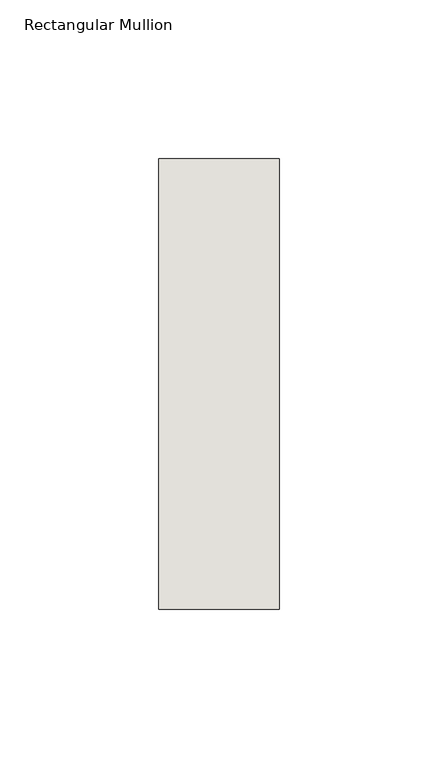
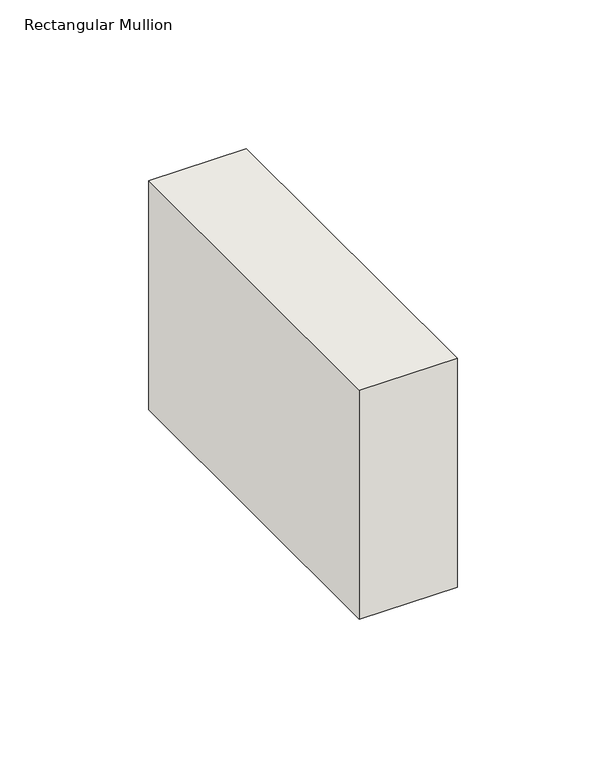
"""IFC4 building model written with IfcOpenShell, lengths in millimetres: wall geometry, Rectangular Mullion : NLRS_21_CWM_hsb-regel 38x142_gen_rsf."""

import ifcopenshell
import ifcopenshell.guid

model = None  # the IFC model being written
_history = None  # IfcOwnerHistory: only IFC2X3 demands one
_inside = {}  # id of a spatial element -> (the spatial element, [elements in it])
_under = {}  # id of a project, library or spatial element -> (it, [spatial elements below it])
_declared = {}  # id of a project -> (the project, [libraries it declares])
_typed = {}  # id of a type object -> (the type object, [elements of that type])
_made_of = {}  # id of a material, layer set ... -> (it, [elements and type objects made of it])


def new_model(schema):
    """Start an empty IFC model of exactly this schema.

    Asked for "IFC4X3", IfcOpenShell would pick the latest addendum, in which some entities
    have other attributes; the version numbers below select the first issue.
    IFC2X3 requires an IfcOwnerHistory on every rooted entity: one is made here for all.
    """
    global model, _history
    if schema == "IFC4X3":
        model = ifcopenshell.file(schema_version=(4, 3, 0, 0))
    else:
        model = ifcopenshell.file(schema=schema)
    _inside.clear()
    _under.clear()
    _declared.clear()
    _typed.clear()
    _made_of.clear()
    _history = None
    if model.schema == "IFC2X3":
        org = make("IfcOrganization", Name="unknown")
        user = make(
            "IfcPersonAndOrganization",
            ThePerson=make("IfcPerson", FamilyName="unknown"),
            TheOrganization=org,
        )
        app = make(
            "IfcApplication",
            ApplicationDeveloper=org,
            Version="unknown",
            ApplicationFullName="unknown",
            ApplicationIdentifier="unknown",
        )
        _history = make(
            "IfcOwnerHistory",
            OwningUser=user,
            OwningApplication=app,
            ChangeAction="ADDED",
            CreationDate=0,
        )
    return model


def make(cls, **values):
    """One entity of the class cls with the attributes given. An attribute that is None is left unset."""
    return model.create_entity(
        cls, **{name: value for name, value in values.items() if value is not None}
    )


def rooted(cls, **values):
    """An entity with a GlobalId (a new one), such as an element, a storey or a relation."""
    return make(cls, GlobalId=ifcopenshell.guid.new(), OwnerHistory=_history, **values)


def si_unit(unit_type, name, prefix=None):
    """IfcSIUnit, for example si_unit("LENGTHUNIT", "METRE", prefix="MILLI")."""
    return make("IfcSIUnit", UnitType=unit_type, Prefix=prefix, Name=name)


def assignment(units):
    """IfcUnitAssignment: the units of a project."""
    return None if units is None else make("IfcUnitAssignment", Units=units)


def point(xyz):
    """IfcCartesianPoint."""
    return None if xyz is None else make("IfcCartesianPoint", Coordinates=xyz)


def direction(xyz):
    """IfcDirection."""
    return None if xyz is None else make("IfcDirection", DirectionRatios=xyz)


def frame(location, z_axis=None, x_axis=None):
    """IfcAxis2Placement3D, a coordinate frame: its origin and axes. An axis left out is left unset."""
    return make(
        "IfcAxis2Placement3D",
        Location=point(location),
        Axis=direction(z_axis),
        RefDirection=direction(x_axis),
    )


def origin():
    """The frame at (0, 0, 0) with its axes left unset."""
    return frame((0.0, 0.0, 0.0))


def place(relative_to, where):
    """IfcLocalPlacement: puts the frame where relative to a parent placement (None: the world)."""
    return make(
        "IfcLocalPlacement", PlacementRelTo=relative_to, RelativePlacement=where
    )


def context(
    kind, dimensions, precision=None, world=None, true_north=None, identifier=None
):
    """IfcGeometricRepresentationContext, for example the 3D "Model" context."""
    return make(
        "IfcGeometricRepresentationContext",
        ContextIdentifier=identifier,
        ContextType=kind,
        CoordinateSpaceDimension=dimensions,
        Precision=precision,
        WorldCoordinateSystem=world,
        TrueNorth=true_north,
    )


def project(units=None, contexts=None):
    """IfcProject with its units and contexts."""
    return rooted(
        "IfcProject",
        Name="project",
        RepresentationContexts=contexts,
        UnitsInContext=assignment(units),
    )


def spatial(cls, under=None, at=None, **own):
    """A site, building, storey or space (cls), placed at a placement, below another one or the project."""
    s = rooted(cls, ObjectPlacement=at, **own)
    if under is not None:
        _under.setdefault(under.id(), (under, []))[1].append(s)
    return s


def polyline(points):
    """IfcPolyline through the points."""
    return make("IfcPolyline", Points=[point(p) for p in points])


def outline(outer, holes=None, kind="AREA"):
    """IfcArbitraryClosedProfileDef: a profile drawn as a closed curve; with holes, ...WithVoids."""
    if holes is None:
        return make("IfcArbitraryClosedProfileDef", ProfileType=kind, OuterCurve=outer)
    return make(
        "IfcArbitraryProfileDefWithVoids",
        ProfileType=kind,
        OuterCurve=outer,
        InnerCurves=holes,
    )


def extrude(swept, where, along, depth):
    """IfcExtrudedAreaSolid: the profile swept, set in the frame where, extruded along a direction by depth."""
    return make(
        "IfcExtrudedAreaSolid",
        SweptArea=swept,
        Position=where,
        ExtrudedDirection=direction(along),
        Depth=depth,
    )


def shape(context_of_items, identifier, shape_type, items):
    """IfcShapeRepresentation: the items that make up one representation, for example the "Body"."""
    return make(
        "IfcShapeRepresentation",
        ContextOfItems=context_of_items,
        RepresentationIdentifier=identifier,
        RepresentationType=shape_type,
        Items=items,
    )


def source(mapping_origin, context_of_items, identifier, shape_type, items):
    """IfcRepresentationMap: a shape defined once, which mapped items show again and again."""
    return make(
        "IfcRepresentationMap",
        MappingOrigin=mapping_origin,
        MappedRepresentation=shape(context_of_items, identifier, shape_type, items),
    )


def transform(
    local_origin,
    x_axis=None,
    y_axis=None,
    z_axis=None,
    scale=None,
    scale2=None,
    scale3=None,
    uniform=True,
):
    """IfcCartesianTransformationOperator3D, or its non-uniform kind. x_axis, y_axis, z_axis: its Axis1, 2, 3."""
    if uniform:
        return make(
            "IfcCartesianTransformationOperator3D",
            Axis1=direction(x_axis),
            Axis2=direction(y_axis),
            LocalOrigin=point(local_origin),
            Scale=scale,
            Axis3=direction(z_axis),
        )
    return make(
        "IfcCartesianTransformationOperator3DnonUniform",
        Axis1=direction(x_axis),
        Axis2=direction(y_axis),
        LocalOrigin=point(local_origin),
        Scale=scale,
        Axis3=direction(z_axis),
        Scale2=scale2,
        Scale3=scale3,
    )


def mapped(mapping_source, mapping_target):
    """IfcMappedItem: shows the shape of a source again, moved by a transform."""
    return make(
        "IfcMappedItem", MappingSource=mapping_source, MappingTarget=mapping_target
    )


def made_of(thing, what):
    """Note that an element or type object is made of a material, layer set ...; save() writes the relation."""
    if what is not None:
        _made_of.setdefault(what.id(), (what, []))[1].append(thing)
    return thing


def element(
    cls,
    number,
    at=None,
    inside=None,
    cuts=None,
    type_object=None,
    material=None,
    context=None,
    identifier="Body",
    shape_type=None,
    held_by="IfcProductDefinitionShape",
    body=None,
    shapes=None,
    **own,
):
    """One element of the class cls, such as IfcWall. Its Tag is "e" and its number.

    at: its placement. inside: the storey or other place that contains it. cuts: it is an
    opening in that element (IfcRelVoidsElement). A single representation is given by context,
    identifier, shape_type and body (its items); several are given by shapes. held_by: the class
    of the entity that holds the representations. save() writes the other relations.
    """
    e = rooted(cls, Tag="e%d" % number, ObjectPlacement=at, **own)
    if body is not None:
        shapes = [shape(context, identifier, shape_type, body)]
    if shapes is not None:
        e.Representation = make(held_by, Representations=shapes)
    if inside is not None:
        _inside.setdefault(inside.id(), (inside, []))[1].append(e)
    if cuts is not None:
        rooted(
            "IfcRelVoidsElement", RelatingBuildingElement=cuts, RelatedOpeningElement=e
        )
    if type_object is not None:
        _typed.setdefault(type_object.id(), (type_object, []))[1].append(e)
    return made_of(e, material)


def aggregate(whole, parts):
    """IfcRelAggregates: a whole, such as a stair, and the parts it consists of."""
    return rooted("IfcRelAggregates", RelatingObject=whole, RelatedObjects=parts)


def save(model, path):
    """Write the relations noted so far, then the file.

    IfcRelAggregates (storeys below a building ...), IfcRelContainedInSpatialStructure (elements
    in a storey), IfcRelDefinesByType, IfcRelAssociatesMaterial and IfcRelDeclares: one each for
    every whole, place, type object, material and project.
    """
    for whole, parts in _under.values():
        aggregate(whole, parts)
    for where, things in _inside.values():
        rooted(
            "IfcRelContainedInSpatialStructure",
            RelatedElements=things,
            RelatingStructure=where,
        )
    for kind, things in _typed.values():
        rooted("IfcRelDefinesByType", RelatedObjects=things, RelatingType=kind)
    for what, things in _made_of.values():
        rooted("IfcRelAssociatesMaterial", RelatedObjects=things, RelatingMaterial=what)
    for by, libraries in _declared.values():
        rooted("IfcRelDeclares", RelatingContext=by, RelatedDefinitions=libraries)
    model.write(path)


def rectangular_mullion_06bc030d(model_context):
    return source(origin(), model_context, "Body", "SweptSolid", [
        extrude(outline(polyline([(19.0, -71.0), (-19.0, -71.0), (-19.0, 71.0), (19.0, 71.0), (19.0, -71.0)])), frame((0.0, 0.0, -94.1558939), z_axis=(0.0, 0.0, 1.0), x_axis=(1.0, 0.0, 0.0)), (0.0, 0.0, 1.0), 94.1558939),
    ])


if __name__ == "__main__":
    model = new_model("IFC4")
    model_context = context("Model", 3, world=origin())
    ifc_project = project(units=[si_unit("LENGTHUNIT", "METRE", prefix="MILLI")], contexts=[model_context])
    site = spatial("IfcSite", under=ifc_project)
    building = spatial("IfcBuilding", under=site)
    placement = place(None, origin())
    rectangular_mullion_shape = rectangular_mullion_06bc030d(model_context)
    element("IfcWall", 1, ObjectType="Rectangular Mullion : NLRS_21_CWM_hsb-regel 38x142_gen_rsf", at=placement, inside=building, context=model_context, shape_type="MappedRepresentation", body=[
        mapped(rectangular_mullion_shape, transform((0.0, 0.0, 0.0), x_axis=(1.0, 0.0, 0.0), y_axis=(0.0, 1.0, 0.0), z_axis=(0.0, 0.0, 1.0))),
    ])
    save(model, "model.ifc")

# Revit data of these elements
# Type "Rectangular Mullion : NLRS_21_CWM_hsb-regel 38x142_gen_rsf"
#   Type IfcGUID = "07M7mRoiH1CR8m_RSKIwpF"
#   Assembly Code = "21.10"
#   IfcExportAs = "IfcWall"
#   built-in parameter 1007322 = 0.465879 (stored number, unit not read)
#   built-in parameter 1007321 = 0.062336 (stored number, unit not read)
#   built-in parameter 1007320 = 0.062336 (stored number, unit not read)
# Element 1 (IfcWall, "Rectangular Mullion : NLRS_21_CWM_hsb-regel 38x142_gen_rsf")
#   Materials on its faces: "NLRS_i2_hout naaldhout vuren_gen_rsf"
# Materials
#   "NLRS_i2_hout naaldhout vuren_gen_rsf": class "I - Hout", colour RGB 234 199 147, transparency 0, Keynote = "i2", Manufacturer = "Revit Standards Foundation", URL = "www.revitstandards.org", Description = "hout vuren", Cost = 0
